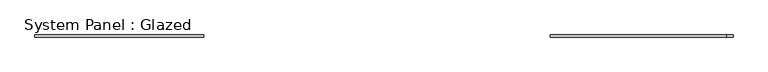
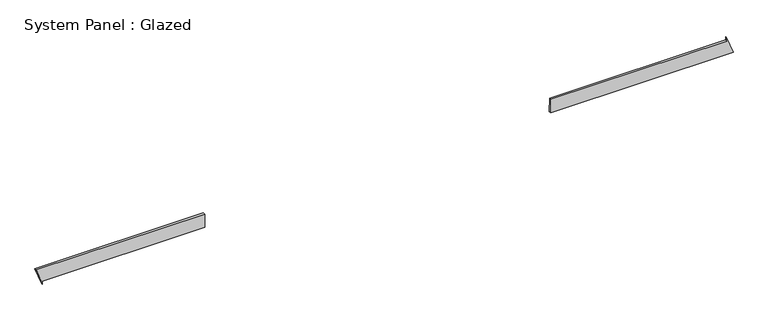
"""IFC4 building model written with IfcOpenShell, lengths in millimetres: plate geometry, System Panel : Glazed."""

from ifc_helpers import new_model, si_unit, frame, origin, place, context, project, spatial, polyline, outline, extrude, source, transform, mapped, element, save


def system_panel_glazed_641e3d16(model_context):
    return source(origin(), model_context, "Body", "SweptSolid", [
        extrude(outline(polyline([(0.0, -3957.2941299), (35.3553391, -3957.2941299), (35.3553391, -2080.9817209), (198.4286437, -2081.9508043), (198.5124481, -4028.0649835), (0.0, -3957.2941299)])), frame((0.0, -49.5, 0.0), z_axis=(0.0, 1.0, 0.0), x_axis=(0.0, 0.0, 1.0)), (0.0, 0.0, 1.0), 25.0),
        extrude(outline(polyline([(35.3553391, 1920.0844805), (35.3553391, 4028.0649835), (233.5239524, 3956.4980838), (198.1686134, 3956.4965613), (198.2562684, 1920.9642368), (35.3553391, 1920.0844805)])), frame((0.0, -49.5, 0.0), z_axis=(0.0, 1.0, 0.0), x_axis=(0.0, 0.0, 1.0)), (0.0, 0.0, 1.0), 25.0),
    ])


if __name__ == "__main__":
    model = new_model("IFC4")
    model_context = context("Model", 3, world=origin())
    ifc_project = project(units=[si_unit("LENGTHUNIT", "METRE", prefix="MILLI")], contexts=[model_context])
    site = spatial("IfcSite", under=ifc_project)
    building = spatial("IfcBuilding", under=site)
    placement = place(None, origin())
    system_panel_glazed_shape = system_panel_glazed_641e3d16(model_context)
    element("IfcPlate", 1, ObjectType="System Panel : Glazed", at=placement, inside=building, context=model_context, shape_type="MappedRepresentation", body=[
        mapped(system_panel_glazed_shape, transform((0.0, 0.0, 0.0), x_axis=(1.0, 0.0, 0.0), y_axis=(0.0, 1.0, 0.0), z_axis=(0.0, 0.0, 1.0))),
    ])
    save(model, "model.ifc")

# Revit data of these elements
# Element 1 (IfcPlate, "System Panel : Glazed")
#   Materials on its faces: "Glass"
# Materials
#   "Glass": class "Glass", colour RGB 218 227 224, transparency 0.85, Description = "Soda Lime Glass", Cost = 0
